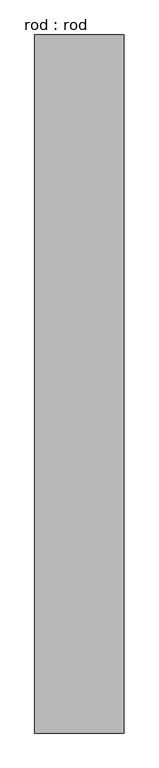
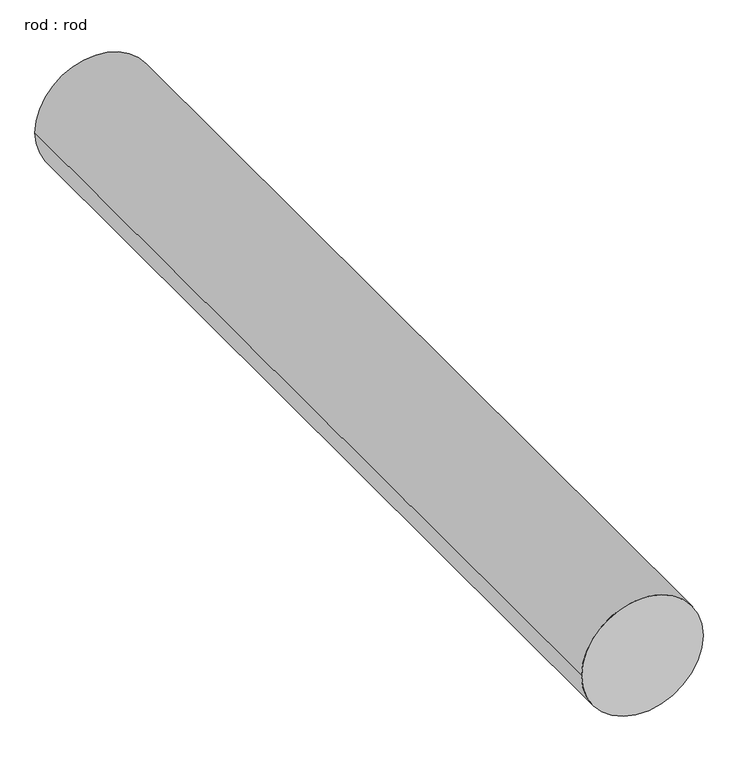
"""IFC4 building model written with IfcOpenShell, lengths in millimetres: proxy geometry, rod : rod."""

from ifc_helpers import new_model, si_unit, point, frame, frame_2d, origin, place, context, project, spatial, circle_curve, trimmed, segment, composite_curve, outline, extrude, source, transform, mapped, element, save


def rod_rod_bc0eaf5b(model_context):
    return source(origin(), model_context, "Body", "SweptSolid", [
        extrude(outline(composite_curve([segment(trimmed(circle_curve(frame_2d((0.0108462, 0.0)), 200.0), [point((0.0108462, 200.0))], [point((0.0108462, -200.0))], False, "CARTESIAN"), True, "CONTINUOUS"), segment(trimmed(circle_curve(frame_2d((0.0108462, 0.0)), 200.0), [point((0.0108462, -200.0))], [point((0.0108462, 200.0))], False, "CARTESIAN"), True, "CONTINUOUS")], self_intersect=False)), frame((0.0, 2532.7286153, 0.0), z_axis=(0.0, 1.0, 0.0), x_axis=(0.0, 0.0, 1.0)), (0.0, 0.0, 1.0), 3120.0),
    ])


if __name__ == "__main__":
    model = new_model("IFC4")
    model_context = context("Model", 3, world=origin())
    ifc_project = project(units=[si_unit("LENGTHUNIT", "METRE", prefix="MILLI")], contexts=[model_context])
    site = spatial("IfcSite", under=ifc_project)
    building = spatial("IfcBuilding", under=site)
    placement = place(None, origin())
    rod_rod_shape = rod_rod_bc0eaf5b(model_context)
    element("IfcBuildingElementProxy", 1, Name="rod : rod", ObjectType="rod : rod", at=placement, inside=building, context=model_context, shape_type="MappedRepresentation", body=[
        mapped(rod_rod_shape, transform((0.0, 0.0, 0.0), x_axis=(1.0, 0.0, 0.0), y_axis=(0.0, 1.0, 0.0), z_axis=(0.0, 0.0, 1.0))),
    ])
    save(model, "model.ifc")

# Revit data of these elements
# Type "rod : rod"
#   Default Elevation = 0
